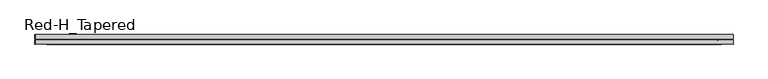
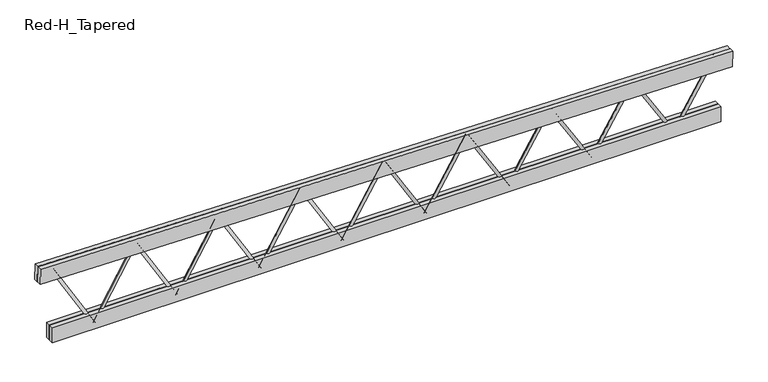
"""IFC4 building model written with IfcOpenShell, lengths in millimetres: beam geometry, Construction_Frames_RedBuilt_Openweb_Red-H_Tapered : Red-H_Tapered."""

from ifc_helpers import new_model, si_unit, point, frame, origin, origin_2d, place, context, project, spatial, polyline, circle_curve, trimmed, segment, composite_curve, outline, extrude, source, transform, mapped, element, save


def red_h_tapered_2af9aea2(model_context):
    return source(origin(), model_context, "Body", "SweptSolid", [
        extrude(outline(composite_curve([segment(trimmed(circle_curve(origin_2d(), 12.7), [point((0.0, 12.7))], [point((0.0, -12.6999999))], False, "CARTESIAN"), True, "CONTINUOUS"), segment(trimmed(circle_curve(origin_2d(), 12.7), [point((0.0, -12.6999999))], [point((0.0, 12.7))], False, "CARTESIAN"), True, "CONTINUOUS")], self_intersect=False)), frame((2516.98125, 0.0, -367.0101562), z_axis=(0.5241619828542637, 0.0, 0.8516185858295288), x_axis=(0.0, -1.0, 0.0)), (0.0, 0.0, 1.0), 685.9878468),
        extrude(outline(composite_curve([segment(trimmed(circle_curve(origin_2d(), 12.7), [point((0.0, -12.7))], [point((0.0, 12.7))], False, "CARTESIAN"), True, "CONTINUOUS"), segment(trimmed(circle_curve(origin_2d(), 12.7), [point((0.0, 12.7))], [point((0.0, -12.7))], False, "CARTESIAN"), True, "CONTINUOUS")], self_intersect=False)), frame((2516.98125, 0.0, -367.0101562), z_axis=(-0.5215905305106932, 0.0, 0.8531959437793724), x_axis=(0.0, -1.0, 0.0)), (0.0, 0.0, 1.0), 689.3697814),
        extrude(outline(composite_curve([segment(trimmed(circle_curve(origin_2d(), 12.7), [point((0.0, 12.7))], [point((0.0, -12.7))], False, "CARTESIAN"), True, "CONTINUOUS"), segment(trimmed(circle_curve(origin_2d(), 12.7), [point((0.0, -12.7))], [point((0.0, 12.7))], False, "CARTESIAN"), True, "CONTINUOUS")], self_intersect=False)), frame((1797.84375, 0.0, -367.0101562), z_axis=(0.5215905305106924, 0.0, 0.8531959437793728), x_axis=(0.0, -1.0, 0.0)), (0.0, 0.0, 1.0), 689.3697814),
        extrude(outline(composite_curve([segment(trimmed(circle_curve(origin_2d(), 12.7), [point((0.0, -12.7))], [point((0.0, 12.7))], False, "CARTESIAN"), True, "CONTINUOUS"), segment(trimmed(circle_curve(origin_2d(), 12.7), [point((0.0, 12.7))], [point((0.0, -12.7))], False, "CARTESIAN"), True, "CONTINUOUS")], self_intersect=False)), frame((1797.84375, 0.0, -367.0101562), z_axis=(-0.519039530732917, 0.0, 0.8547502357627949), x_axis=(0.0, -1.0, 0.0)), (0.0, 0.0, 1.0), 692.7579283),
        extrude(outline(composite_curve([segment(trimmed(circle_curve(origin_2d(), 12.7), [point((0.0, 12.7))], [point((0.0, -12.7))], False, "CARTESIAN"), True, "CONTINUOUS"), segment(trimmed(circle_curve(origin_2d(), 12.7), [point((0.0, -12.7))], [point((0.0, 12.7))], False, "CARTESIAN"), True, "CONTINUOUS")], self_intersect=False)), frame((1078.70625, 0.0, -367.0101562), z_axis=(0.519039530732916, 0.0, 0.8547502357627954), x_axis=(0.0, -1.0, 0.0)), (0.0, 0.0, 1.0), 692.7579283),
        extrude(outline(composite_curve([segment(trimmed(circle_curve(origin_2d(), 12.7), [point((0.0, -12.7))], [point((0.0, 12.7))], False, "CARTESIAN"), True, "CONTINUOUS"), segment(trimmed(circle_curve(origin_2d(), 12.7), [point((0.0, 12.7))], [point((0.0, -12.7))], False, "CARTESIAN"), True, "CONTINUOUS")], self_intersect=False)), frame((1078.70625, 0.0, -367.0101562), z_axis=(-0.5165088204868722, 0.0, 0.8562818685218438), x_axis=(0.0, -1.0, 0.0)), (0.0, 0.0, 1.0), 696.1521967),
        extrude(outline(composite_curve([segment(trimmed(circle_curve(origin_2d(), 12.7), [point((0.0, 12.7))], [point((0.0, -12.7))], False, "CARTESIAN"), True, "CONTINUOUS"), segment(trimmed(circle_curve(origin_2d(), 12.7), [point((0.0, -12.7))], [point((0.0, 12.7))], False, "CARTESIAN"), True, "CONTINUOUS")], self_intersect=False)), frame((359.56875, 0.0, -367.0101562), z_axis=(0.5165088204868726, 0.0, 0.8562818685218435), x_axis=(0.0, -1.0, 0.0)), (0.0, 0.0, 1.0), 696.1521967),
        extrude(outline(composite_curve([segment(trimmed(circle_curve(origin_2d(), 12.7), [point((0.0, -12.7000001))], [point((0.0, 12.7))], False, "CARTESIAN"), True, "CONTINUOUS"), segment(trimmed(circle_curve(origin_2d(), 12.7), [point((0.0, 12.7))], [point((0.0, -12.7000001))], False, "CARTESIAN"), True, "CONTINUOUS")], self_intersect=False)), frame((359.56875, 0.0, -367.0101562), z_axis=(-0.513998236342516, 0.0, 0.8577912409419807), x_axis=(0.0, -1.0, 0.0)), (0.0, 0.0, 1.0), 699.5524976),
        extrude(outline(composite_curve([segment(trimmed(circle_curve(origin_2d(), 12.7), [point((0.0, -12.7))], [point((0.0, 12.7000001))], False, "CARTESIAN"), True, "CONTINUOUS"), segment(trimmed(circle_curve(origin_2d(), 12.7), [point((0.0, 12.7000001))], [point((0.0, -12.7))], False, "CARTESIAN"), True, "CONTINUOUS")], self_intersect=False)), frame((-359.56875, 0.0, -367.0101562), z_axis=(0.5139982363424845, 0.0, 0.8577912409419995), x_axis=(0.0, -1.0, 0.0)), (0.0, 0.0, 1.0), 699.5524976),
        extrude(outline(composite_curve([segment(trimmed(circle_curve(origin_2d(), 12.7), [point((0.0, 12.7))], [point((0.0, -12.7000001))], False, "CARTESIAN"), True, "CONTINUOUS"), segment(trimmed(circle_curve(origin_2d(), 12.7), [point((0.0, -12.7000001))], [point((0.0, 12.7))], False, "CARTESIAN"), True, "CONTINUOUS")], self_intersect=False)), frame((-359.56875, 0.0, -367.0101562), z_axis=(-0.511507614574279, 0.0, 0.8592787441991865), x_axis=(0.0, -1.0, 0.0)), (0.0, 0.0, 1.0), 702.9587434),
        extrude(outline(composite_curve([segment(trimmed(circle_curve(origin_2d(), 12.7), [point((0.0, -12.7))], [point((0.0, 12.7000001))], False, "CARTESIAN"), True, "CONTINUOUS"), segment(trimmed(circle_curve(origin_2d(), 12.7), [point((0.0, 12.7000001))], [point((0.0, -12.7))], False, "CARTESIAN"), True, "CONTINUOUS")], self_intersect=False)), frame((-1078.70625, 0.0, -367.0101562), z_axis=(0.5115076145742774, 0.0, 0.8592787441991874), x_axis=(0.0, -1.0, 0.0)), (0.0, 0.0, 1.0), 702.9587434),
        extrude(outline(composite_curve([segment(trimmed(circle_curve(origin_2d(), 12.7), [point((0.0, 12.7))], [point((0.0, -12.7))], False, "CARTESIAN"), True, "CONTINUOUS"), segment(trimmed(circle_curve(origin_2d(), 12.7), [point((0.0, -12.7))], [point((0.0, 12.7))], False, "CARTESIAN"), True, "CONTINUOUS")], self_intersect=False)), frame((-1078.70625, 0.0, -367.0101562), z_axis=(-0.5090367912567517, 0.0, 0.8607447619050784), x_axis=(0.0, -1.0, 0.0)), (0.0, 0.0, 1.0), 706.3708482),
        extrude(outline(composite_curve([segment(trimmed(circle_curve(origin_2d(), 12.7), [point((0.0, -12.7))], [point((0.0, 12.7))], False, "CARTESIAN"), True, "CONTINUOUS"), segment(trimmed(circle_curve(origin_2d(), 12.7), [point((0.0, 12.7))], [point((0.0, -12.7))], False, "CARTESIAN"), True, "CONTINUOUS")], self_intersect=False)), frame((-1797.84375, 0.0, -367.0101562), z_axis=(0.5090367912567648, 0.0, 0.8607447619050707), x_axis=(0.0, -1.0, 0.0)), (0.0, 0.0, 1.0), 706.3708482),
        extrude(outline(composite_curve([segment(trimmed(circle_curve(origin_2d(), 12.7), [point((0.0, 12.7))], [point((0.0, -12.7))], False, "CARTESIAN"), True, "CONTINUOUS"), segment(trimmed(circle_curve(origin_2d(), 12.7), [point((0.0, -12.7))], [point((0.0, 12.7))], False, "CARTESIAN"), True, "CONTINUOUS")], self_intersect=False)), frame((-1797.84375, 0.0, -367.0101562), z_axis=(-0.5065856023552368, 0.0, 0.8621896702503353), x_axis=(0.0, -1.0, 0.0)), (0.0, 0.0, 1.0), 709.7887274),
        extrude(outline(composite_curve([segment(trimmed(circle_curve(origin_2d(), 12.7), [point((0.0, -12.7))], [point((0.0, 12.7))], False, "CARTESIAN"), True, "CONTINUOUS"), segment(trimmed(circle_curve(origin_2d(), 12.7), [point((0.0, 12.7))], [point((0.0, -12.7))], False, "CARTESIAN"), True, "CONTINUOUS")], self_intersect=False)), frame((-2516.98125, 0.0, -367.0101562), z_axis=(0.5065856023552251, 0.0, 0.8621896702503422), x_axis=(0.0, -1.0, 0.0)), (0.0, 0.0, 1.0), 709.7887274),
        extrude(outline(composite_curve([segment(trimmed(circle_curve(origin_2d(), 12.7), [point((0.0, 12.6999999))], [point((0.0, -12.7))], False, "CARTESIAN"), True, "CONTINUOUS"), segment(trimmed(circle_curve(origin_2d(), 12.7), [point((0.0, -12.7))], [point((0.0, 12.6999999))], False, "CARTESIAN"), True, "CONTINUOUS")], self_intersect=False)), frame((-2516.98125, 0.0, -367.0101562), z_axis=(-0.5041538838118749, 0.0, 0.8636138381460794), x_axis=(0.0, -1.0, 0.0)), (0.0, 0.0, 1.0), 713.212298),
        extrude(outline(polyline([(-2901.95, -41.275), (-2901.95, -3.175), (2901.95, -3.175), (2901.95, -41.275), (-2901.95, -41.275)])), frame((0.0, 0.0, -386.0601562), z_axis=(0.0, 0.0, 1.0), x_axis=(1.0, 0.0, 0.0)), (0.0, 0.0, 1.0), 139.7),
        extrude(outline(polyline([(-2901.95, 3.175), (-2901.95, 41.275), (2901.95, 41.275), (2901.95, 3.175), (-2901.95, 3.175)])), frame((0.0, 0.0, -386.0601562), z_axis=(0.0, 0.0, 1.0), x_axis=(1.0, 0.0, 0.0)), (0.0, 0.0, 1.0), 139.7),
        extrude(outline(polyline([(0.0, -38.1), (0.0, 0.0), (6007.9591352, 0.0), (6007.9591352, -38.1), (0.0, -38.1)])), frame((-3005.9124528, -3.175, 185.4598208), z_axis=(0.01691090064262469, 0.0, 0.9998570004952985), x_axis=(0.9998570004952985, 0.0, -0.01691090064262469)), (0.0, 0.0, 1.0), 139.7),
        extrude(outline(polyline([(0.0, -38.1), (0.0, 0.0), (6007.9591352, 0.0), (6007.9591352, -38.1), (0.0, -38.1)])), frame((-3005.9124528, 41.275, 185.4598208), z_axis=(0.01691090064262469, 0.0, 0.9998570004952985), x_axis=(0.9998570004952985, 0.0, -0.01691090064262469)), (0.0, 0.0, 1.0), 139.7),
    ])


if __name__ == "__main__":
    model = new_model("IFC4")
    model_context = context("Model", 3, world=origin())
    ifc_project = project(units=[si_unit("LENGTHUNIT", "METRE", prefix="MILLI")], contexts=[model_context])
    site = spatial("IfcSite", under=ifc_project)
    building = spatial("IfcBuilding", under=site)
    placement = place(None, origin())
    red_h_tapered_shape = red_h_tapered_2af9aea2(model_context)
    element("IfcBeam", 1, ObjectType="Construction_Frames_RedBuilt_Openweb_Red-H_Tapered : Red-H_Tapered", at=placement, inside=building, context=model_context, shape_type="MappedRepresentation", body=[
        mapped(red_h_tapered_shape, transform((0.0, 0.0, 0.0), x_axis=(1.0, 0.0, 0.0), y_axis=(0.0, 1.0, 0.0), z_axis=(0.0, 0.0, 1.0))),
    ])
    save(model, "model.ifc")

# Revit data of these elements
# Type "Construction_Frames_RedBuilt_Openweb_Red-H_Tapered : Red-H_Tapered"
#   Youtube clip = ""
#   Weight Net (Kg) = "0"
#   Webs = "Up to 2\" diameter tubular steel"
#   Uniformat II Description = ""
#   Uniformat II Code = ""
#   Uniclass 2015 Name = "Softwood trusses"
#   Uniclass 2015 Code = "Pr_20_85_90_81"
#   Uniclass 2.0 Description = "Structural Framing Systems"
#   Uniclass 2.0 Code = "SS-15-10-75"
#   Uniclass 1.4 Description = "Trusses"
#   Uniclass 1.4 Code = "L3523"
#   UNSPSC Code = "30103606"
#   Technical description = "http://www.redbuilt.com/reference/literature-and-other-resources"
#   Region South America = "None"
#   Region Oceania = "None"
#   Region North America = "US"
#   Region Middle East = "None"
#   Region Europe = "None"
#   Region Asia = "None"
#   Region Antarctica = "None"
#   Region Africa = "None"
#   QR code = "http://bimobject.com/redbuilt/product/redbuilt-0003"
#   Product url = "http://www.redbuilt.com/products/default.aspx?id=2"
#   Product group = "Wood Trusses"
#   Product family = "Construction"
#   Product data url = "https://bimobject.com/redbuilt/product/redbuilt-0003"
#   Product certification = ""
#   Product SKU = "redbuilt-0003"
#   Product Page URL = "http://www.redbuilt.com/commercial-systems/red-m-red-h-open-web-trusses"
#   Product Guid = "2c5793f2-6ffb-4665-b825-cf90c048e711"
#   Product Documentation Link = "http://www.redbuilt.com/documents/OW_Guide_2017_07_LowRes_wLinks.pdf"
#   OmniClass Description = "Wood Trusses"
#   OmniClass Code = "23-13 35 19 13 17"
#   NBS Reference Description = ""
#   NBS Reference Code = ""
#   Material secondary = "Steel"
#   Material main = "CHARRED WOOD"
#   Masterformat 2014 Description = "Metal-Web Wood Joists"
#   Masterformat 2014 Code = "06 17 36"
#   Manufacturer name = "RedBuilt"
#   Manufacturer country = "United States"
#   Installation instructions = "http://www.redbuilt.com/documents/Installation_Sheets_Open-Web.pdf"
#   IFC Classification = ""
#   EAN code = ""
#   Design country = "United States"
#   Product Information = "http://redbuilt.com/products/default.aspx?id=2"
#   Model = "Red-H-Tapered"
#   Manufacturer URL = "http://redbuilt.com/"
#   Manufacturer = "RedBuilt™"
#   Description = "Open Web Truss"
#   Date of publishing = "8/17/2010"
#   Contact us = "http://redbuilt.com/contact/"
#   Chords = "Double 1½\" x 5½\" MSR lumber"
#   COBIe Type Category = ""
#   Brand url = "http://www.redbuilt.com"
#   BIMobject main category code = "construction"
#   BIMobject main category = "Construction"
#   BIMobject category code = "construction-frames-trusses"
#   BIMobject category = "Frames & Trusses"
#   Web Radius = 0' - 0 1/2"
#   Web Layout Offset Start [instance default] = 0' - 5"
#   Web Layout Offset End [instance default] = 0' - 5"
#   Web Diameter = 0' - 1"
#   TotalLength [instance default] = 20' - 0"
#   Span Minimum = 4' - 0"
#   Span Maximum = 70' - 0"
#   Span Limit [instance default] = 20' - 0"
#   Nominal width = 0' - 0"
#   Nominal height = 0' - 0"
#   Inner Depth Top [instance default] = 0' - 2.76372"
#   Depth Start [instance default] = 6' - 0"
#   Top Chord Length [instance default] = 20' - 1.19701"
#   TC Extension Start Aux [instance default] = 0' - 0"
#   TC Extension End Aux [instance default] = 0' - 0"
#   T-B Chord Length Difference L [instance default] = 0' - 4"
#   T-B Chord Length Difference [instance default] = 0' - 4"
#   Height 2 [instance default] = 6' - 0"
#   Depth Minimum at Wall = 2' - 0"
#   Depth Maximum at Wall = 6' - 0"
#   Depth Lower End [instance default] = 2' - 0"
#   Depth Higher End [instance default] = 6' - 0"
#   Depth End [instance default] = 2' - 0"
#   Depth 2 [instance default] = 2' - 0"
#   Chord Width = 0' - 3 1/4"
#   Chord Thickness = 0' - 1 1/2"
#   Chord Depth = 0' - 5 1/2"
#   Offset Start [instance default] = 0' - 0"
#   TC Extension Start [instance default] = 0' - 0"
#   End Panel = 0' - 5"
#   Offset End [instance default] = 0' - 0"
#   TC Extension End [instance default] = 0' - 0"
#   Length [instance default] = 20' - 0"
#   Angle [instance default] = 5.71059°
#   Span Limit Warning [instance default] = no
#   Edition number = 1
#   Top Bearing Start [instance default] = yes
#   Top Bearing End [instance default] = yes
#   Bottom Bearing Start [instance default] = no
#   Bottom Bearing End [instance default] = no
#   8 Panels [instance default] = yes
#   16 Panels [instance default] = no
#   12 Panels [instance default] = no
#   Web Material = RedBuilt-Steel, Galvanized
#   Clip Material = RedBuilt-Steel, Galvanized
#   Chords Material = WOOD-OAKFIRE
#   URL = ""
#   Assembly Code = ""
# Element 1 (IfcBeam, "Construction_Frames_RedBuilt_Openweb_Red-H_Tapered : Red-H_Tapered")
#   TotalLength = 19' - 8 1/2"
#   Span Limit = 19' - 8 1/2"
#   Inner Depth Top = 0' - 2.75039"
#   Depth Start = 5' - 0"
#   Top Chord Length = 19' - 8.53382"
#   Height 2 = 5' - 0"
#   Depth Higher End = 5' - 0"
#   Depth 2 = 0' - 4"
#   Angle = 0.968969°
#   Materials on its faces: "RedBuilt-Steel, Galvanized", "WOOD-OAKFIRE"
# Materials
#   "RedBuilt-Steel, Galvanized": class "Metal", colour RGB 164 172 176, transparency 0, Manufacturer = "RedBuilt. LLC", Comments = "Openweb Metal Web", URL = "http://www.redbuilt.com/", Description = "Galvanized steel", Cost = 0
#   "WOOD-OAKFIRE": class "Wood", colour RGB 198 202 183, transparency 0, Description = "Generic wood", Cost = 0
